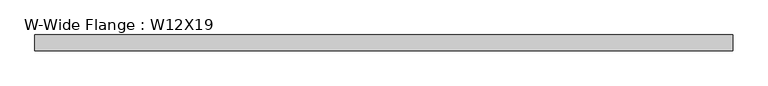
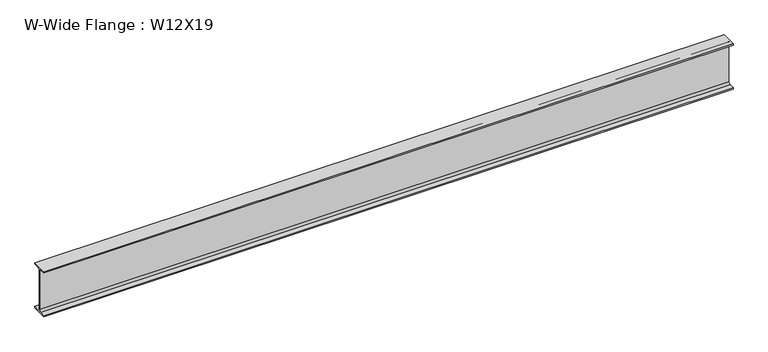
"""IFC4 building model written with IfcOpenShell, lengths in millimetres: beam geometry, W-Wide Flange : W12X19."""

import ifcopenshell
import ifcopenshell.guid

model = None  # the IFC model being written
_history = None  # IfcOwnerHistory: only IFC2X3 demands one
_inside = {}  # id of a spatial element -> (the spatial element, [elements in it])
_under = {}  # id of a project, library or spatial element -> (it, [spatial elements below it])
_declared = {}  # id of a project -> (the project, [libraries it declares])
_typed = {}  # id of a type object -> (the type object, [elements of that type])
_made_of = {}  # id of a material, layer set ... -> (it, [elements and type objects made of it])


def new_model(schema):
    """Start an empty IFC model of exactly this schema.

    Asked for "IFC4X3", IfcOpenShell would pick the latest addendum, in which some entities
    have other attributes; the version numbers below select the first issue.
    IFC2X3 requires an IfcOwnerHistory on every rooted entity: one is made here for all.
    """
    global model, _history
    if schema == "IFC4X3":
        model = ifcopenshell.file(schema_version=(4, 3, 0, 0))
    else:
        model = ifcopenshell.file(schema=schema)
    _inside.clear()
    _under.clear()
    _declared.clear()
    _typed.clear()
    _made_of.clear()
    _history = None
    if model.schema == "IFC2X3":
        org = make("IfcOrganization", Name="unknown")
        user = make(
            "IfcPersonAndOrganization",
            ThePerson=make("IfcPerson", FamilyName="unknown"),
            TheOrganization=org,
        )
        app = make(
            "IfcApplication",
            ApplicationDeveloper=org,
            Version="unknown",
            ApplicationFullName="unknown",
            ApplicationIdentifier="unknown",
        )
        _history = make(
            "IfcOwnerHistory",
            OwningUser=user,
            OwningApplication=app,
            ChangeAction="ADDED",
            CreationDate=0,
        )
    return model


def make(cls, **values):
    """One entity of the class cls with the attributes given. An attribute that is None is left unset."""
    return model.create_entity(
        cls, **{name: value for name, value in values.items() if value is not None}
    )


def rooted(cls, **values):
    """An entity with a GlobalId (a new one), such as an element, a storey or a relation."""
    return make(cls, GlobalId=ifcopenshell.guid.new(), OwnerHistory=_history, **values)


def si_unit(unit_type, name, prefix=None):
    """IfcSIUnit, for example si_unit("LENGTHUNIT", "METRE", prefix="MILLI")."""
    return make("IfcSIUnit", UnitType=unit_type, Prefix=prefix, Name=name)


def assignment(units):
    """IfcUnitAssignment: the units of a project."""
    return None if units is None else make("IfcUnitAssignment", Units=units)


def point(xyz):
    """IfcCartesianPoint."""
    return None if xyz is None else make("IfcCartesianPoint", Coordinates=xyz)


def direction(xyz):
    """IfcDirection."""
    return None if xyz is None else make("IfcDirection", DirectionRatios=xyz)


def frame(location, z_axis=None, x_axis=None):
    """IfcAxis2Placement3D, a coordinate frame: its origin and axes. An axis left out is left unset."""
    return make(
        "IfcAxis2Placement3D",
        Location=point(location),
        Axis=direction(z_axis),
        RefDirection=direction(x_axis),
    )


def frame_2d(location, x_axis=None):
    """IfcAxis2Placement2D, a coordinate frame in the plane: its origin and x axis."""
    return make(
        "IfcAxis2Placement2D", Location=point(location), RefDirection=direction(x_axis)
    )


def origin():
    """The frame at (0, 0, 0) with its axes left unset."""
    return frame((0.0, 0.0, 0.0))


def place(relative_to, where):
    """IfcLocalPlacement: puts the frame where relative to a parent placement (None: the world)."""
    return make(
        "IfcLocalPlacement", PlacementRelTo=relative_to, RelativePlacement=where
    )


def context(
    kind, dimensions, precision=None, world=None, true_north=None, identifier=None
):
    """IfcGeometricRepresentationContext, for example the 3D "Model" context."""
    return make(
        "IfcGeometricRepresentationContext",
        ContextIdentifier=identifier,
        ContextType=kind,
        CoordinateSpaceDimension=dimensions,
        Precision=precision,
        WorldCoordinateSystem=world,
        TrueNorth=true_north,
    )


def project(units=None, contexts=None):
    """IfcProject with its units and contexts."""
    return rooted(
        "IfcProject",
        Name="project",
        RepresentationContexts=contexts,
        UnitsInContext=assignment(units),
    )


def spatial(cls, under=None, at=None, **own):
    """A site, building, storey or space (cls), placed at a placement, below another one or the project."""
    s = rooted(cls, ObjectPlacement=at, **own)
    if under is not None:
        _under.setdefault(under.id(), (under, []))[1].append(s)
    return s


def polyline(points):
    """IfcPolyline through the points."""
    return make("IfcPolyline", Points=[point(p) for p in points])


def circle_curve(where, radius):
    """IfcCircle in the frame where."""
    return make("IfcCircle", Position=where, Radius=radius)


def trimmed(basis, trim1, trim2, sense, master):
    """IfcTrimmedCurve: the piece of a basis curve between two trims."""
    return make(
        "IfcTrimmedCurve",
        BasisCurve=basis,
        Trim1=trim1,
        Trim2=trim2,
        SenseAgreement=sense,
        MasterRepresentation=master,
    )


def segment(curve, same_sense, transition):
    """IfcCompositeCurveSegment."""
    return make(
        "IfcCompositeCurveSegment",
        Transition=transition,
        SameSense=same_sense,
        ParentCurve=curve,
    )


def composite_curve(segments, self_intersect=None):
    """IfcCompositeCurve: segments joined end to end."""
    return make("IfcCompositeCurve", Segments=segments, SelfIntersect=self_intersect)


def outline(outer, holes=None, kind="AREA"):
    """IfcArbitraryClosedProfileDef: a profile drawn as a closed curve; with holes, ...WithVoids."""
    if holes is None:
        return make("IfcArbitraryClosedProfileDef", ProfileType=kind, OuterCurve=outer)
    return make(
        "IfcArbitraryProfileDefWithVoids",
        ProfileType=kind,
        OuterCurve=outer,
        InnerCurves=holes,
    )


def extrude(swept, where, along, depth):
    """IfcExtrudedAreaSolid: the profile swept, set in the frame where, extruded along a direction by depth."""
    return make(
        "IfcExtrudedAreaSolid",
        SweptArea=swept,
        Position=where,
        ExtrudedDirection=direction(along),
        Depth=depth,
    )


def shape(context_of_items, identifier, shape_type, items):
    """IfcShapeRepresentation: the items that make up one representation, for example the "Body"."""
    return make(
        "IfcShapeRepresentation",
        ContextOfItems=context_of_items,
        RepresentationIdentifier=identifier,
        RepresentationType=shape_type,
        Items=items,
    )


def source(mapping_origin, context_of_items, identifier, shape_type, items):
    """IfcRepresentationMap: a shape defined once, which mapped items show again and again."""
    return make(
        "IfcRepresentationMap",
        MappingOrigin=mapping_origin,
        MappedRepresentation=shape(context_of_items, identifier, shape_type, items),
    )


def transform(
    local_origin,
    x_axis=None,
    y_axis=None,
    z_axis=None,
    scale=None,
    scale2=None,
    scale3=None,
    uniform=True,
):
    """IfcCartesianTransformationOperator3D, or its non-uniform kind. x_axis, y_axis, z_axis: its Axis1, 2, 3."""
    if uniform:
        return make(
            "IfcCartesianTransformationOperator3D",
            Axis1=direction(x_axis),
            Axis2=direction(y_axis),
            LocalOrigin=point(local_origin),
            Scale=scale,
            Axis3=direction(z_axis),
        )
    return make(
        "IfcCartesianTransformationOperator3DnonUniform",
        Axis1=direction(x_axis),
        Axis2=direction(y_axis),
        LocalOrigin=point(local_origin),
        Scale=scale,
        Axis3=direction(z_axis),
        Scale2=scale2,
        Scale3=scale3,
    )


def mapped(mapping_source, mapping_target):
    """IfcMappedItem: shows the shape of a source again, moved by a transform."""
    return make(
        "IfcMappedItem", MappingSource=mapping_source, MappingTarget=mapping_target
    )


def made_of(thing, what):
    """Note that an element or type object is made of a material, layer set ...; save() writes the relation."""
    if what is not None:
        _made_of.setdefault(what.id(), (what, []))[1].append(thing)
    return thing


def element(
    cls,
    number,
    at=None,
    inside=None,
    cuts=None,
    type_object=None,
    material=None,
    context=None,
    identifier="Body",
    shape_type=None,
    held_by="IfcProductDefinitionShape",
    body=None,
    shapes=None,
    **own,
):
    """One element of the class cls, such as IfcWall. Its Tag is "e" and its number.

    at: its placement. inside: the storey or other place that contains it. cuts: it is an
    opening in that element (IfcRelVoidsElement). A single representation is given by context,
    identifier, shape_type and body (its items); several are given by shapes. held_by: the class
    of the entity that holds the representations. save() writes the other relations.
    """
    e = rooted(cls, Tag="e%d" % number, ObjectPlacement=at, **own)
    if body is not None:
        shapes = [shape(context, identifier, shape_type, body)]
    if shapes is not None:
        e.Representation = make(held_by, Representations=shapes)
    if inside is not None:
        _inside.setdefault(inside.id(), (inside, []))[1].append(e)
    if cuts is not None:
        rooted(
            "IfcRelVoidsElement", RelatingBuildingElement=cuts, RelatedOpeningElement=e
        )
    if type_object is not None:
        _typed.setdefault(type_object.id(), (type_object, []))[1].append(e)
    return made_of(e, material)


def aggregate(whole, parts):
    """IfcRelAggregates: a whole, such as a stair, and the parts it consists of."""
    return rooted("IfcRelAggregates", RelatingObject=whole, RelatedObjects=parts)


def save(model, path):
    """Write the relations noted so far, then the file.

    IfcRelAggregates (storeys below a building ...), IfcRelContainedInSpatialStructure (elements
    in a storey), IfcRelDefinesByType, IfcRelAssociatesMaterial and IfcRelDeclares: one each for
    every whole, place, type object, material and project.
    """
    for whole, parts in _under.values():
        aggregate(whole, parts)
    for where, things in _inside.values():
        rooted(
            "IfcRelContainedInSpatialStructure",
            RelatedElements=things,
            RelatingStructure=where,
        )
    for kind, things in _typed.values():
        rooted("IfcRelDefinesByType", RelatedObjects=things, RelatingType=kind)
    for what, things in _made_of.values():
        rooted("IfcRelAssociatesMaterial", RelatedObjects=things, RelatingMaterial=what)
    for by, libraries in _declared.values():
        rooted("IfcRelDeclares", RelatingContext=by, RelatedDefinitions=libraries)
    model.write(path)


def w_wide_flange_w12x19_50e300ca(model_context):
    return source(origin(), model_context, "Body", "SweptSolid", [
        extrude(outline(composite_curve([segment(polyline([(50.927, -146.05), (50.927, -154.94), (-50.927, -154.94), (-50.927, -146.05), (-16.3195, -146.05)]), True, "CONTINUOUS"), segment(trimmed(circle_curve(frame_2d((-16.3195, -132.715)), 13.335), [point((-16.3195, -146.05))], [point((-2.9845, -132.715))], True, "CARTESIAN"), True, "CONTINUOUS"), segment(polyline([(-2.9845, -132.715), (-2.9845, 132.715)]), True, "CONTINUOUS"), segment(trimmed(circle_curve(frame_2d((-16.3195, 132.715)), 13.335), [point((-2.9845, 132.715))], [point((-16.3195, 146.05))], True, "CARTESIAN"), True, "CONTINUOUS"), segment(polyline([(-16.3195, 146.05), (-50.927, 146.05), (-50.927, 154.94), (50.927, 154.94), (50.927, 146.05), (16.3195, 146.05)]), True, "CONTINUOUS"), segment(trimmed(circle_curve(frame_2d((16.3195, 132.715)), 13.335), [point((16.3195, 146.05))], [point((2.9845, 132.715))], True, "CARTESIAN"), True, "CONTINUOUS"), segment(polyline([(2.9845, 132.715), (2.9845, -132.715)]), True, "CONTINUOUS"), segment(trimmed(circle_curve(frame_2d((16.3195, -132.715)), 13.335), [point((2.9845, -132.715))], [point((16.3195, -146.05))], True, "CARTESIAN"), True, "CONTINUOUS"), segment(polyline([(16.3195, -146.05), (50.927, -146.05)]), True, "CONTINUOUS")], self_intersect=False)), frame((-2235.2, 0.0, 0.0), z_axis=(1.0, 0.0, 0.0), x_axis=(0.0, 1.0, 0.0)), (0.0, 0.0, 1.0), 4470.4),
    ])


if __name__ == "__main__":
    model = new_model("IFC4")
    model_context = context("Model", 3, world=origin())
    ifc_project = project(units=[si_unit("LENGTHUNIT", "METRE", prefix="MILLI")], contexts=[model_context])
    site = spatial("IfcSite", under=ifc_project)
    building = spatial("IfcBuilding", under=site)
    placement = place(None, origin())
    w_wide_flange_w12x19_shape = w_wide_flange_w12x19_50e300ca(model_context)
    element("IfcBeam", 1, ObjectType="W-Wide Flange : W12X19", at=placement, inside=building, context=model_context, shape_type="MappedRepresentation", body=[
        mapped(w_wide_flange_w12x19_shape, transform((0.0, 0.0, 0.0), x_axis=(1.0, 0.0, 0.0), y_axis=(0.0, 1.0, 0.0), z_axis=(0.0, 0.0, 1.0))),
    ])
    save(model, "model.ifc")

# Revit data of these elements
# Type "W-Wide Flange : W12X19"
#   Assembly Code = "B10"
#   W = 19
#   Length [instance default] = 5' - 0"
#   bf = 0' - 4.01"
#   d = 1' - 0.2"
#   k = 0' - 0 7/8"
#   k2 = 0' - 0.525"
#   tf = 0' - 0.35"
#   tw = 0' - 0.235"
#   A = 0.0386806 SF
#   Structural Material [instance default] = Steel ASTM A992
# Element 1 (IfcBeam, "W-Wide Flange : W12X19")
#   Materials on its faces: "Steel ASTM A992"
# Materials
#   "Steel ASTM A992": class "Metal", colour RGB 199 199 199, transparency 0, Description = "Structural steel 50ksi", Cost = 0
